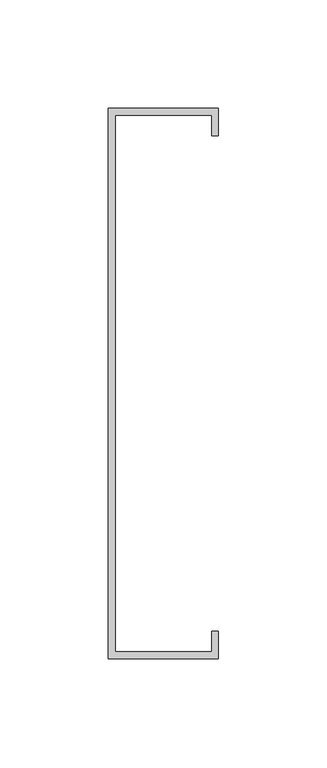
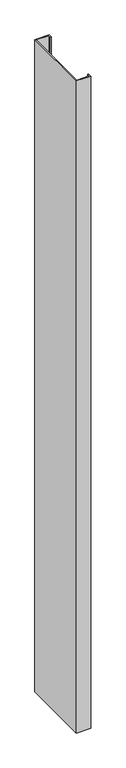
"""IFC4 building model written with IfcOpenShell, lengths in millimetres: proxy geometry, Generic Models 2:Generic Models 2:310765:Generic Models 2:310765 : Generic Models 2:Generic Models 2:310765:63 : Generic Models 2:Generic Models 2:310765:Generic Models 2:310765 : Generic Models 2:Generic Models 2:310765:300385."""

from ifc_helpers import new_model, si_unit, origin, origin_with_axes, place, context, project, spatial, polyline, outline, extrude, source, transform, mapped, element, save


def generic_models_4e90fef1(model_context):
    return source(origin(), model_context, "Body", "SweptSolid", [
        extrude(outline(polyline([(593798.4117242, -536557.2913358), (593849.2117242, -536557.2913358), (593849.2117242, -536569.9913358), (593846.0367242, -536569.9913358), (593846.0367242, -536560.4663358), (593801.5867242, -536560.4663358), (593801.5867242, -536808.1163358), (593846.0367242, -536808.1163358), (593846.0367242, -536798.5913358), (593849.2117242, -536798.5913358), (593849.2117242, -536811.2913358), (593798.4117242, -536811.2913358), (593798.4117242, -536557.2913358)])), origin_with_axes(), (0.0, 0.0, 1.0), 2438.255317),
    ])


if __name__ == "__main__":
    model = new_model("IFC4")
    model_context = context("Model", 3, world=origin())
    ifc_project = project(units=[si_unit("LENGTHUNIT", "METRE", prefix="MILLI")], contexts=[model_context])
    site = spatial("IfcSite", under=ifc_project)
    building = spatial("IfcBuilding", under=site)
    placement = place(None, origin())
    generic_models_shape = generic_models_4e90fef1(model_context)
    element("IfcBuildingElementProxy", 1, Name="Generic Models 2:Generic Models 2:310765:Generic Models 2:310765 : Generic Models 2:Generic Models 2:310765:63 : Generic Models 2:Generic Models 2:310765:Generic Models 2:310765 : Generic Models 2:Generic Models 2:310765:300385", ObjectType="Generic Models 2:Generic Models 2:310765:Generic Models 2:310765 : Generic Models 2:Generic Models 2:310765:63 : Generic Models 2:Generic Models 2:310765:Generic Models 2:310765 : Generic Models 2:Generic Models 2:310765:300385", at=placement, inside=building, context=model_context, shape_type="MappedRepresentation", body=[
        mapped(generic_models_shape, transform((0.0, 0.0, 0.0), x_axis=(1.0, 0.0, 0.0), y_axis=(0.0, 1.0, 0.0), z_axis=(0.0, 0.0, 1.0))),
    ])
    save(model, "model.ifc")

# Revit data of these elements
# Type "Generic Models 2:Generic Models 2:310765:Generic Models 2:310765 : Generic Models 2:Generic Models 2:310765:63 : Generic Models 2:Generic Models 2:310765:Generic Models 2:310765 : Generic Models 2:Generic Models 2:310765:300385"
#   NameOverride = "Generic Models 2:Generic Models 2:310765:Generic Models 2:310765 : Generic Models 2:Generic Models 2:310765:300385"
#   ObjectTypeOverride = "Generic Models 2:310765 : Generic Models 2:Generic Models 2:310765"
#   Reference = "Generic Models 2"
#   Tag = "300385"
# Element 1 (IfcBuildingElementProxy, "Generic Models 2:Generic Models 2:310765:Generic Models 2:310765 : Generic Models 2:Generic Models 2:310765:63 : Generic Models 2:Generic Models 2:310765:Generic Models 2:310765 : Generic Models 2:Generic Models 2:310765:300385")
#   Materials on its faces: "STRUCTURAL STEEL - SEE STRUCT. DWGS"
# Materials
#   "STRUCTURAL STEEL - SEE STRUCT. DWGS": class "Metal", colour RGB 189 187 185, transparency 0, Description = "Structural steel 50ksi", Cost = 0
